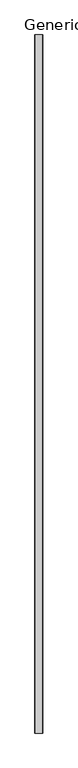
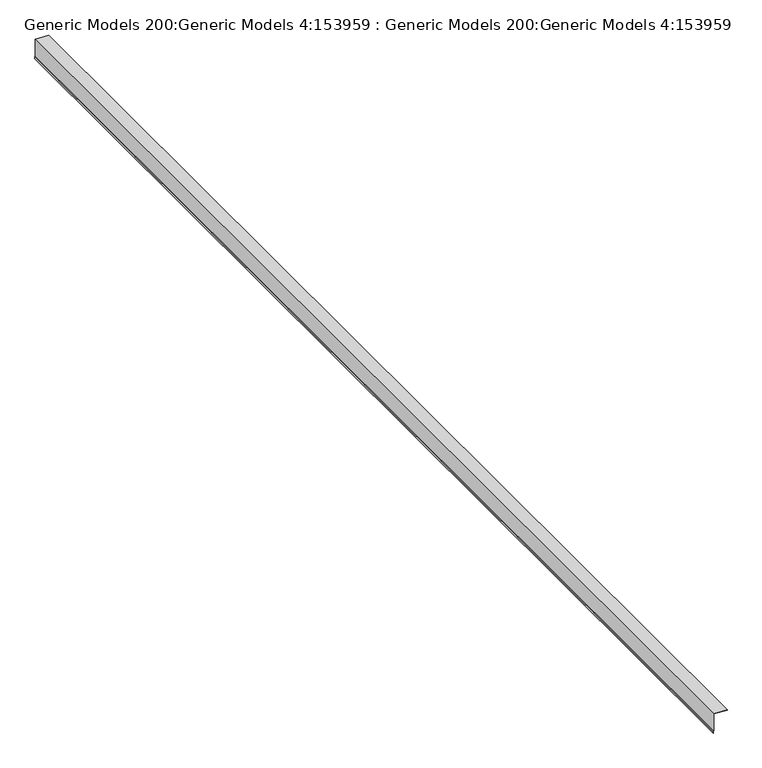
"""IFC4 building model written with IfcOpenShell, lengths in millimetres: proxy geometry, Generic Models 200:Generic Models 4:153959 : Generic Models 200:Generic Models 4:153959."""

from ifc_helpers import new_model, si_unit, frame, origin, place, context, project, spatial, polyline, outline, extrude, source, transform, mapped, element, save


def generic_models_200_generic_models_4_153959_generic_models_c056b5f2(model_context):
    return source(origin(), model_context, "Body", "SweptSolid", [
        extrude(outline(polyline([(3395.4425401, -8390.6330237), (3414.4765001, -8390.6330237), (3421.6084406, -8388.0372097), (3633.6961326, -8388.0372097), (3627.1165517, -8230.1272689), (3627.9123721, -8230.1604281), (3634.5236442, -8388.8309597), (3421.7484002, -8388.8309597), (3414.6164596, -8391.4267737), (3395.4425401, -8391.4267737), (3395.4425401, -8390.6330237)])), frame((0.0, -6674.7974793, 0.0), z_axis=(0.0, 1.0, 0.0), x_axis=(0.0, 0.0, 1.0)), (0.0, 0.0, 1.0), 13919.2),
    ])


if __name__ == "__main__":
    model = new_model("IFC4")
    model_context = context("Model", 3, world=origin())
    ifc_project = project(units=[si_unit("LENGTHUNIT", "METRE", prefix="MILLI")], contexts=[model_context])
    site = spatial("IfcSite", under=ifc_project)
    building = spatial("IfcBuilding", under=site)
    placement = place(None, origin())
    generic_models_200_generic_models_4_153959_generic_models_shape = generic_models_200_generic_models_4_153959_generic_models_c056b5f2(model_context)
    element("IfcBuildingElementProxy", 1, Name="Generic Models 200:Generic Models 4:153959 : Generic Models 200:Generic Models 4:153959", ObjectType="Generic Models 200:Generic Models 4:153959 : Generic Models 200:Generic Models 4:153959", at=placement, inside=building, context=model_context, shape_type="MappedRepresentation", body=[
        mapped(generic_models_200_generic_models_4_153959_generic_models_shape, transform((0.0, 0.0, 0.0), x_axis=(1.0, 0.0, 0.0), y_axis=(0.0, 1.0, 0.0), z_axis=(0.0, 0.0, 1.0))),
    ])
    save(model, "model.ifc")

# Revit data of these elements
# Type "Generic Models 200:Generic Models 4:153959 : Generic Models 200:Generic Models 4:153959"
#   NameOverride = "Generic Models 200:Generic Models 4:153959"
#   ObjectTypeOverride = "Generic Models 200:Generic Models 4"
#   Reference = "Generic Models 4"
#   Category = "Generic Models"
#   Tag = "153959"
# Element 1 (IfcBuildingElementProxy, "Generic Models 200:Generic Models 4:153959 : Generic Models 200:Generic Models 4:153959")
#   Materials on its faces: "_(2) LAYERS NO. 30 ASTM D226 ASPHALT SATURATED ORGANIC FELT 997"
# Materials
#   "_(2) LAYERS NO. 30 ASTM D226 ASPHALT SATURATED ORGANIC FELT 997": class "Unassigned", colour RGB 67 154 161, transparency 0
